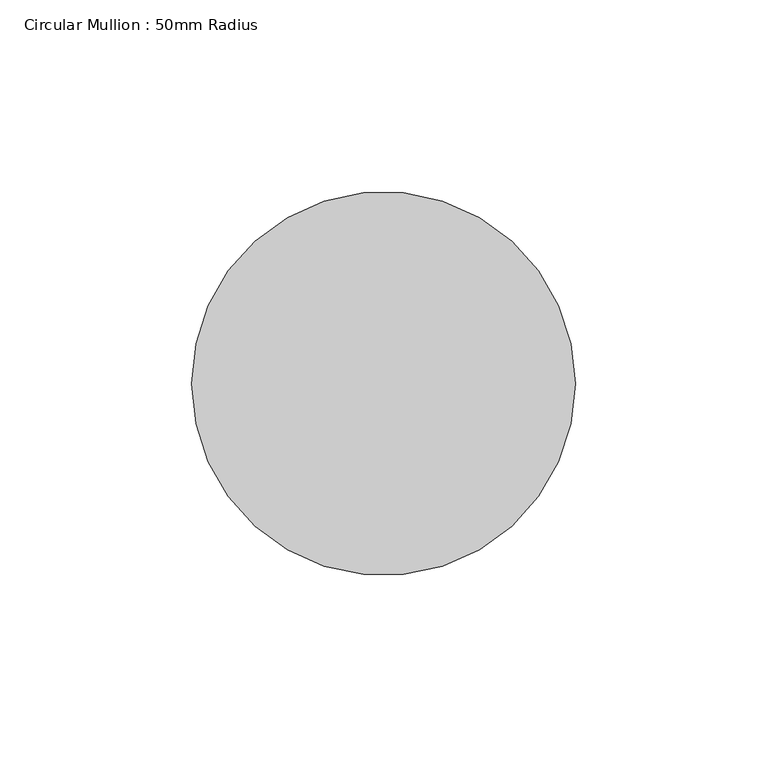
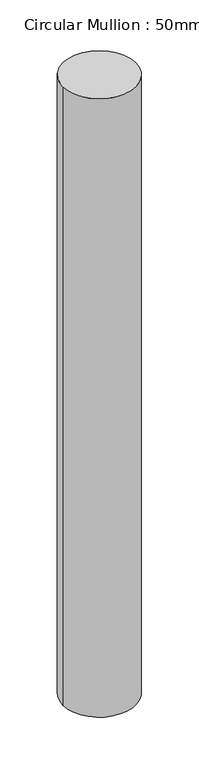
"""IFC4 building model written with IfcOpenShell, lengths in millimetres: member geometry, Circular Mullion : 50mm Radius."""

from ifc_helpers import new_model, si_unit, point, frame, origin, origin_2d, place, context, project, spatial, circle_curve, trimmed, segment, composite_curve, outline, extrude, source, transform, mapped, element, save


def circular_mullion_50mm_radius_b956e016(model_context):
    return source(origin(), model_context, "Body", "SweptSolid", [
        extrude(outline(composite_curve([segment(trimmed(circle_curve(origin_2d(), 50.0), [point((50.0, 0.0))], [point((-50.0, 0.0))], False, "CARTESIAN"), True, "CONTINUOUS"), segment(trimmed(circle_curve(origin_2d(), 50.0), [point((-50.0, 0.0))], [point((50.0, 0.0))], False, "CARTESIAN"), True, "CONTINUOUS")], self_intersect=False)), frame((0.0, 0.0, -899.0700382), z_axis=(0.0, 0.0, 1.0), x_axis=(1.0, 0.0, 0.0)), (0.0, 0.0, 1.0), 899.0700382),
    ])


if __name__ == "__main__":
    model = new_model("IFC4")
    model_context = context("Model", 3, world=origin())
    ifc_project = project(units=[si_unit("LENGTHUNIT", "METRE", prefix="MILLI")], contexts=[model_context])
    site = spatial("IfcSite", under=ifc_project)
    building = spatial("IfcBuilding", under=site)
    placement = place(None, origin())
    circular_mullion_50mm_radius_shape = circular_mullion_50mm_radius_b956e016(model_context)
    element("IfcMember", 1, ObjectType="Circular Mullion : 50mm Radius", at=placement, inside=building, context=model_context, shape_type="MappedRepresentation", body=[
        mapped(circular_mullion_50mm_radius_shape, transform((0.0, 0.0, 0.0), x_axis=(1.0, 0.0, 0.0), y_axis=(0.0, 1.0, 0.0), z_axis=(0.0, 0.0, 1.0))),
    ])
    save(model, "model.ifc")

# Revit data of these elements
# Type "Circular Mullion : 50mm Radius"
#   built-in parameter 1007350 = 0.164042 (stored number, unit not read)
# Element 1 (IfcMember, "Circular Mullion : 50mm Radius")
#   Materials on its faces: "Aluminium"
# Materials
#   "Aluminium": class "Metal", colour RGB 247 247 247, transparency 0, Description = "Aluminium 6061", Cost = 0
